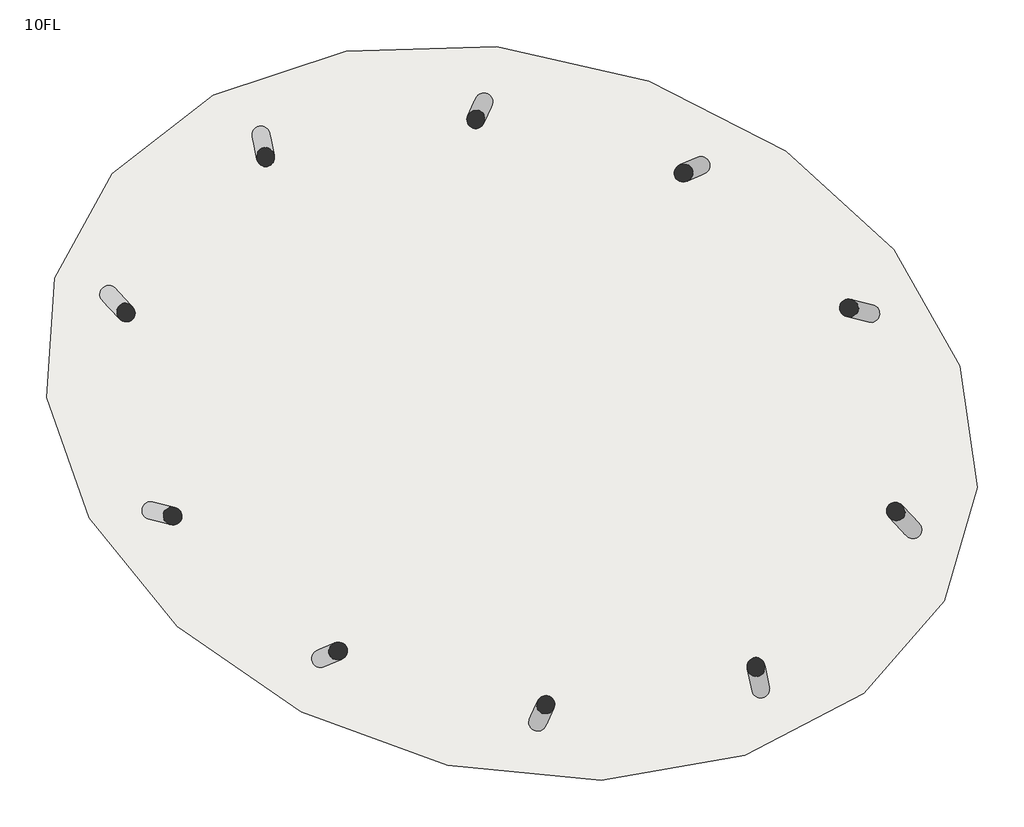
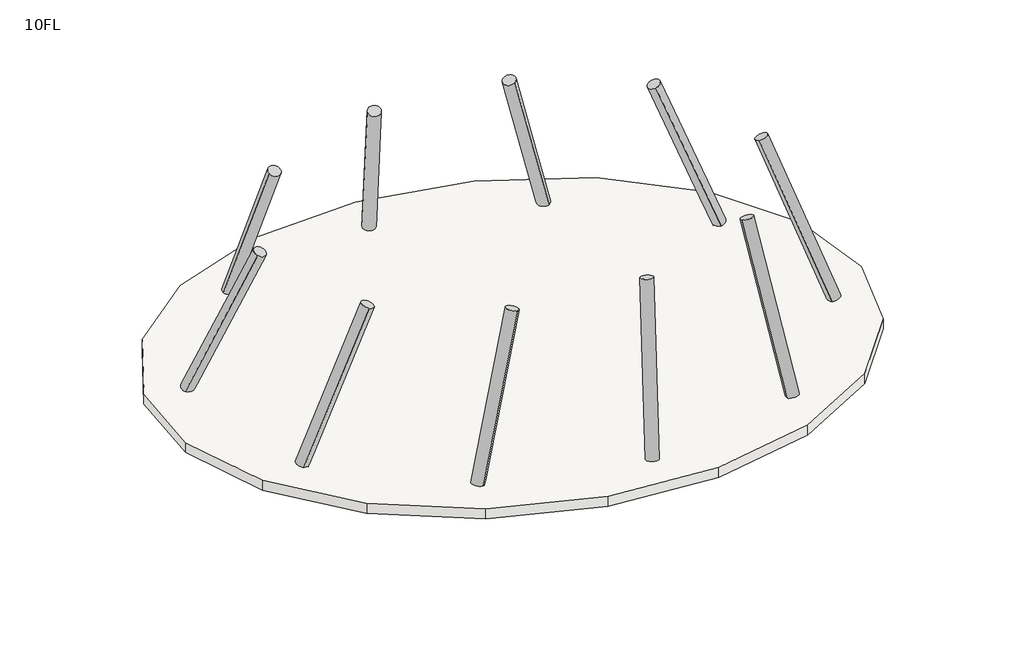
# One storey: 10 columns, 1 slab.
"""IFC4 building model written with IfcOpenShell, lengths in millimetres."""

from ifc_helpers import new_model, si_unit, point, frame, frame_2d, origin, place, context, project, spatial, polyline, circle_curve, trimmed, segment, composite_curve, outline, extrude, element, save

model = new_model("IFC4")

# Units and contexts
model_context = context("Model", 3, world=origin())
ifc_project = project(units=[si_unit("LENGTHUNIT", "METRE", prefix="MILLI")], contexts=[model_context])

# Site, building, storey
site = spatial("IfcSite", under=ifc_project)
building = spatial("IfcBuilding", under=site)
storey = spatial("IfcBuildingStorey", under=building, Name="10FL", Elevation=40500.0)

# Columns
placement = place(None, origin())
element("IfcColumn", 1, ObjectType="コンクリート-円形-柱 : 750", at=placement, inside=storey, context=model_context, shape_type="SweptSolid", body=[
    extrude(outline(composite_curve([segment(trimmed(circle_curve(frame_2d((1e-07, -175.0)), 175.0), [point((1e-07, -350.0))], [point((0.0, 0.0))], False, "CARTESIAN"), True, "CONTINUOUS"), segment(trimmed(circle_curve(frame_2d((1e-07, -175.0)), 175.0), [point((0.0, 0.0))], [point((1e-07, -350.0))], False, "CARTESIAN"), True, "CONTINUOUS")], self_intersect=False)), frame((-7782.3746067, 2442.3902219, 40500.0), z_axis=(0.26401293669722087, -0.28099078546262674, 0.9226816069162784), x_axis=(0.6318034246632209, -0.6724327329372294, -0.38556277343435874)), (0.0, 0.0, 1.0), 4877.088658),
])
element("IfcColumn", 2, ObjectType="コンクリート-円形-柱 : 750", at=placement, inside=storey, context=model_context, shape_type="SweptSolid", body=[
    extrude(outline(composite_curve([segment(trimmed(circle_curve(frame_2d((0.0, -175.0)), 175.0), [point((0.0, -350.0))], [point((0.0, 0.0))], False, "CARTESIAN"), True, "CONTINUOUS"), segment(trimmed(circle_curve(frame_2d((0.0, -175.0)), 175.0), [point((0.0, 0.0))], [point((0.0, -350.0))], False, "CARTESIAN"), True, "CONTINUOUS")], self_intersect=False)), frame((-7040.3567909, -1765.4140721, 40500.0), z_axis=(0.3396986066466646, -0.08649067165219855, 0.9365491019479258), x_axis=(0.9075930761035431, -0.23108229825837925, -0.3505364169962)), (0.0, 0.0, 1.0), 4804.8735412),
])
element("IfcColumn", 3, ObjectType="コンクリート-円形-柱 : 750", at=placement, inside=storey, context=model_context, shape_type="SweptSolid", body=[
    extrude(outline(composite_curve([segment(trimmed(circle_curve(frame_2d((1e-07, -175.0)), 175.0), [point((1e-07, -350.0))], [point((0.0, 0.0))], False, "CARTESIAN"), True, "CONTINUOUS"), segment(trimmed(circle_curve(frame_2d((1e-07, -175.0)), 175.0), [point((0.0, 0.0))], [point((1e-07, -350.0))], False, "CARTESIAN"), True, "CONTINUOUS")], self_intersect=False)), frame((-3812.9513772, -4691.4326676, 40500.0), z_axis=(0.2774723422705273, 0.11970298054053238, 0.953247237459737), x_axis=(0.8752719431856899, 0.37759677063842406, -0.3021915026525063)), (0.0, 0.0, 1.0), 4720.7060489),
])
element("IfcColumn", 4, ObjectType="コンクリート-円形-柱 : 750", at=placement, inside=storey, context=model_context, shape_type="SweptSolid", body=[
    extrude(outline(composite_curve([segment(trimmed(circle_curve(frame_2d((0.0, -175.0)), 175.0), [point((-1e-07, -350.0))], [point((0.0, 0.0))], False, "CARTESIAN"), True, "CONTINUOUS"), segment(trimmed(circle_curve(frame_2d((0.0, -175.0)), 175.0), [point((0.0, 0.0))], [point((-1e-07, -350.0))], False, "CARTESIAN"), True, "CONTINUOUS")], self_intersect=False)), frame((367.1124162, -6032.6694057, 40500.0), z_axis=(0.1272762437041582, 0.27660483194919916, 0.9525179918148083), x_axis=(0.3981607774121528, 0.865308338143962, -0.3044823069885752)), (0.0, 0.0, 1.0), 4724.320213),
])
element("IfcColumn", 5, ObjectType="コンクリート-円形-柱 : 750", at=placement, inside=storey, context=model_context, shape_type="SweptSolid", body=[
    extrude(outline(composite_curve([segment(trimmed(circle_curve(frame_2d((-1e-07, -175.0)), 175.0), [point((0.0, -350.0))], [point((0.0, 0.0))], False, "CARTESIAN"), True, "CONTINUOUS"), segment(trimmed(circle_curve(frame_2d((-1e-07, -175.0)), 175.0), [point((0.0, 0.0))], [point((0.0, -350.0))], False, "CARTESIAN"), True, "CONTINUOUS")], self_intersect=False)), frame((4741.5348144, -5492.9214626, 40500.0), z_axis=(-0.07163495207387421, 0.3463542555471653, 0.9353647220767645), x_axis=(-0.18944787591272252, 0.9159785290157737, -0.3536846571371981)), (0.0, 0.0, 1.0), 4810.9575879),
])
element("IfcColumn", 6, ObjectType="コンクリート-円形-柱 : 750", at=placement, inside=storey, context=model_context, shape_type="SweptSolid", body=[
    extrude(outline(composite_curve([segment(trimmed(circle_curve(frame_2d((0.0, -175.0)), 175.0), [point((0.0, -350.0))], [point((0.0, 0.0))], False, "CARTESIAN"), True, "CONTINUOUS"), segment(trimmed(circle_curve(frame_2d((0.0, -175.0)), 175.0), [point((0.0, 0.0))], [point((0.0, -350.0))], False, "CARTESIAN"), True, "CONTINUOUS")], self_intersect=False)), frame((7782.3746289, -2442.3901937, 40500.0), z_axis=(-0.26401293796979214, 0.2809907859765056, 0.922681606395654), x_axis=(-0.6318034253104986, 0.672432731614684, -0.3855627746802532)), (0.0, 0.0, 1.0), 4877.088658),
])
element("IfcColumn", 7, ObjectType="コンクリート-円形-柱 : 750", at=placement, inside=storey, context=model_context, shape_type="SweptSolid", body=[
    extrude(outline(composite_curve([segment(trimmed(circle_curve(frame_2d((0.0, -175.0000001)), 175.0), [point((0.0, -350.0))], [point((0.0, 0.0))], False, "CARTESIAN"), True, "CONTINUOUS"), segment(trimmed(circle_curve(frame_2d((0.0, -175.0000001)), 175.0), [point((0.0, 0.0))], [point((0.0, -350.0))], False, "CARTESIAN"), True, "CONTINUOUS")], self_intersect=False)), frame((7040.356751, 1765.4140787, 40500.0), z_axis=(-0.3396986042201518, 0.08649067440309391, 0.9365491025740075), x_axis=(-0.9075930745581908, 0.2310823068653006, -0.35053641532346014)), (0.0, 0.0, 1.0), 4804.8735412),
])
element("IfcColumn", 8, ObjectType="コンクリート-円形-柱 : 750", at=placement, inside=storey, context=model_context, shape_type="SweptSolid", body=[
    extrude(outline(composite_curve([segment(trimmed(circle_curve(frame_2d((0.0, -175.0)), 175.0), [point((0.0, -350.0))], [point((0.0, 0.0))], False, "CARTESIAN"), True, "CONTINUOUS"), segment(trimmed(circle_curve(frame_2d((0.0, -175.0)), 175.0), [point((0.0, 0.0))], [point((0.0, -350.0))], False, "CARTESIAN"), True, "CONTINUOUS")], self_intersect=False)), frame((3812.9513461, 4691.4326624, 40500.0), z_axis=(-0.2774723428201125, -0.11970298092490453, 0.9532472372514961), x_axis=(-0.8752719428255081, -0.3775967709476215, -0.3021915033093917)), (0.0, 0.0, 1.0), 4720.7060489),
])
element("IfcColumn", 9, ObjectType="コンクリート-円形-柱 : 750", at=placement, inside=storey, context=model_context, shape_type="SweptSolid", body=[
    extrude(outline(composite_curve([segment(trimmed(circle_curve(frame_2d((0.0, -175.0)), 175.0), [point((0.0, -350.0))], [point((0.0, 0.0))], False, "CARTESIAN"), True, "CONTINUOUS"), segment(trimmed(circle_curve(frame_2d((0.0, -175.0)), 175.0), [point((0.0, 0.0))], [point((0.0, -350.0))], False, "CARTESIAN"), True, "CONTINUOUS")], self_intersect=False)), frame((-367.1124224, 6032.6694038, 40500.0), z_axis=(-0.12727624854847108, -0.2766048320148229, 0.9525179911484504), x_axis=(-0.39816078956223655, -0.8653083318197369, -0.3044823090731555)), (0.0, 0.0, 1.0), 4724.320213),
])
element("IfcColumn", 10, ObjectType="コンクリート-円形-柱 : 750", at=placement, inside=storey, context=model_context, shape_type="SweptSolid", body=[
    extrude(outline(composite_curve([segment(trimmed(circle_curve(frame_2d((0.0, -175.0)), 175.0), [point((0.0, -350.0))], [point((0.0, 0.0))], False, "CARTESIAN"), True, "CONTINUOUS"), segment(trimmed(circle_curve(frame_2d((0.0, -175.0)), 175.0), [point((0.0, 0.0))], [point((0.0, -350.0))], False, "CARTESIAN"), True, "CONTINUOUS")], self_intersect=False)), frame((-4741.5348293, 5492.9214837, 40500.0), z_axis=(0.07163494986715985, -0.3463542608905655, 0.9353647202671692), x_axis=(0.18944786714684828, -0.9159785289808872, -0.35368466192290615)), (0.0, 0.0, 1.0), 4810.9575879),
])

# Slab
element("IfcSlab", 11, ObjectType="一般 300 mm", at=placement, inside=storey, context=model_context, shape_type="SweptSolid", body=[
    extrude(outline(polyline([(-8287.4508866, -2080.1781062), (-9124.1942139, 289.3841433), (-8967.6997676, 2633.1542325), (-7832.2134964, 4689.4663855), (-5847.2181447, 6230.4914027), (-3233.5704394, 7092.7720454), (-274.2297182, 7188.1804065), (2713.3858287, 6509.0016289), (5409.0821673, 5128.5049987), (7523.2055979, 3193.4073339), (8826.2935251, 908.6985374), (9172.017225, -1481.1380999), (8516.7555904, -3712.754224), (6933.8710983, -5536.3004074), (4602.436937, -6753.8172271), (1777.7303523, -7238.7435717), (-1236.3865473, -6942.6877445), (-4116.9204525, -5898.8223862), (-6554.8946324, -4218.619375), (-8287.4508866, -2080.1781062)])), frame((0.0, 0.0, 40200.0), z_axis=(0.0, 0.0, 1.0), x_axis=(1.0, 0.0, 0.0)), (0.0, 0.0, 1.0), 300.0),
])

save(model, "model.ifc")

# Revit data of these elements
# Type "コンクリート-円形-柱 : 750"
#   Keynote = "03310.Q1"
#   R = 350 mm
#   Structural Material [instance default] = コンクリート - 現場打ち
# Type "一般 300 mm"
#   Function = 0
#   Layers, outside or top first: 300 mm no material (function 1)
# Elements 1, 2, 3, 4, 5, 6, 7, 8, 9, 10 (IfcColumn, "コンクリート-円形-柱 : 750")
#   Structural Material = コンクリート - 現場打ち
#   Phase Created = 新しい建設
#   Materials on its faces: "コンクリート - 現場打ち"
# Element 11 (IfcSlab, "一般 300 mm")
#   Height Offset From Level = 0 mm
#   Phase Created = 新しい建設
# Materials
#   "コンクリート - 現場打ち": class "コンクリート", colour RGB 192 192 192, transparency 0
